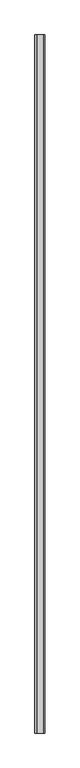
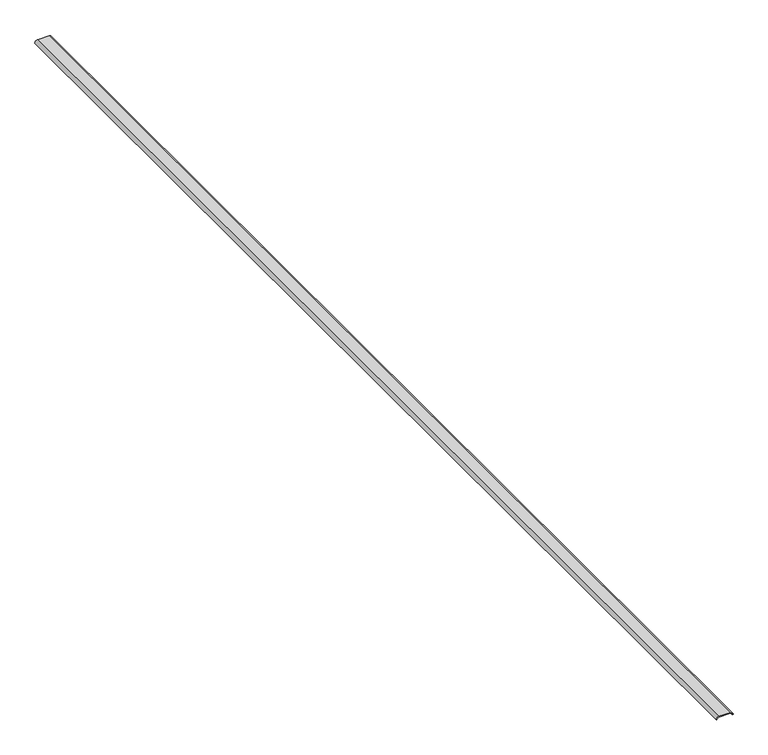
"""IFC4 building model written with IfcOpenShell, lengths in millimetres: proxy geometry, BEND PANEL004 6191 : BEND PANEL004 6191."""

import ifcopenshell
import ifcopenshell.guid

model = None  # the IFC model being written
_history = None  # IfcOwnerHistory: only IFC2X3 demands one
_inside = {}  # id of a spatial element -> (the spatial element, [elements in it])
_under = {}  # id of a project, library or spatial element -> (it, [spatial elements below it])
_declared = {}  # id of a project -> (the project, [libraries it declares])
_typed = {}  # id of a type object -> (the type object, [elements of that type])
_made_of = {}  # id of a material, layer set ... -> (it, [elements and type objects made of it])


def new_model(schema):
    """Start an empty IFC model of exactly this schema.

    Asked for "IFC4X3", IfcOpenShell would pick the latest addendum, in which some entities
    have other attributes; the version numbers below select the first issue.
    IFC2X3 requires an IfcOwnerHistory on every rooted entity: one is made here for all.
    """
    global model, _history
    if schema == "IFC4X3":
        model = ifcopenshell.file(schema_version=(4, 3, 0, 0))
    else:
        model = ifcopenshell.file(schema=schema)
    _inside.clear()
    _under.clear()
    _declared.clear()
    _typed.clear()
    _made_of.clear()
    _history = None
    if model.schema == "IFC2X3":
        org = make("IfcOrganization", Name="unknown")
        user = make(
            "IfcPersonAndOrganization",
            ThePerson=make("IfcPerson", FamilyName="unknown"),
            TheOrganization=org,
        )
        app = make(
            "IfcApplication",
            ApplicationDeveloper=org,
            Version="unknown",
            ApplicationFullName="unknown",
            ApplicationIdentifier="unknown",
        )
        _history = make(
            "IfcOwnerHistory",
            OwningUser=user,
            OwningApplication=app,
            ChangeAction="ADDED",
            CreationDate=0,
        )
    return model


def make(cls, **values):
    """One entity of the class cls with the attributes given. An attribute that is None is left unset."""
    return model.create_entity(
        cls, **{name: value for name, value in values.items() if value is not None}
    )


def rooted(cls, **values):
    """An entity with a GlobalId (a new one), such as an element, a storey or a relation."""
    return make(cls, GlobalId=ifcopenshell.guid.new(), OwnerHistory=_history, **values)


def si_unit(unit_type, name, prefix=None):
    """IfcSIUnit, for example si_unit("LENGTHUNIT", "METRE", prefix="MILLI")."""
    return make("IfcSIUnit", UnitType=unit_type, Prefix=prefix, Name=name)


def assignment(units):
    """IfcUnitAssignment: the units of a project."""
    return None if units is None else make("IfcUnitAssignment", Units=units)


def point(xyz):
    """IfcCartesianPoint."""
    return None if xyz is None else make("IfcCartesianPoint", Coordinates=xyz)


def direction(xyz):
    """IfcDirection."""
    return None if xyz is None else make("IfcDirection", DirectionRatios=xyz)


def frame(location, z_axis=None, x_axis=None):
    """IfcAxis2Placement3D, a coordinate frame: its origin and axes. An axis left out is left unset."""
    return make(
        "IfcAxis2Placement3D",
        Location=point(location),
        Axis=direction(z_axis),
        RefDirection=direction(x_axis),
    )


def frame_2d(location, x_axis=None):
    """IfcAxis2Placement2D, a coordinate frame in the plane: its origin and x axis."""
    return make(
        "IfcAxis2Placement2D", Location=point(location), RefDirection=direction(x_axis)
    )


def origin():
    """The frame at (0, 0, 0) with its axes left unset."""
    return frame((0.0, 0.0, 0.0))


def place(relative_to, where):
    """IfcLocalPlacement: puts the frame where relative to a parent placement (None: the world)."""
    return make(
        "IfcLocalPlacement", PlacementRelTo=relative_to, RelativePlacement=where
    )


def context(
    kind, dimensions, precision=None, world=None, true_north=None, identifier=None
):
    """IfcGeometricRepresentationContext, for example the 3D "Model" context."""
    return make(
        "IfcGeometricRepresentationContext",
        ContextIdentifier=identifier,
        ContextType=kind,
        CoordinateSpaceDimension=dimensions,
        Precision=precision,
        WorldCoordinateSystem=world,
        TrueNorth=true_north,
    )


def project(units=None, contexts=None):
    """IfcProject with its units and contexts."""
    return rooted(
        "IfcProject",
        Name="project",
        RepresentationContexts=contexts,
        UnitsInContext=assignment(units),
    )


def spatial(cls, under=None, at=None, **own):
    """A site, building, storey or space (cls), placed at a placement, below another one or the project."""
    s = rooted(cls, ObjectPlacement=at, **own)
    if under is not None:
        _under.setdefault(under.id(), (under, []))[1].append(s)
    return s


def polyline(points):
    """IfcPolyline through the points."""
    return make("IfcPolyline", Points=[point(p) for p in points])


def circle_curve(where, radius):
    """IfcCircle in the frame where."""
    return make("IfcCircle", Position=where, Radius=radius)


def trimmed(basis, trim1, trim2, sense, master):
    """IfcTrimmedCurve: the piece of a basis curve between two trims."""
    return make(
        "IfcTrimmedCurve",
        BasisCurve=basis,
        Trim1=trim1,
        Trim2=trim2,
        SenseAgreement=sense,
        MasterRepresentation=master,
    )


def segment(curve, same_sense, transition):
    """IfcCompositeCurveSegment."""
    return make(
        "IfcCompositeCurveSegment",
        Transition=transition,
        SameSense=same_sense,
        ParentCurve=curve,
    )


def composite_curve(segments, self_intersect=None):
    """IfcCompositeCurve: segments joined end to end."""
    return make("IfcCompositeCurve", Segments=segments, SelfIntersect=self_intersect)


def outline(outer, holes=None, kind="AREA"):
    """IfcArbitraryClosedProfileDef: a profile drawn as a closed curve; with holes, ...WithVoids."""
    if holes is None:
        return make("IfcArbitraryClosedProfileDef", ProfileType=kind, OuterCurve=outer)
    return make(
        "IfcArbitraryProfileDefWithVoids",
        ProfileType=kind,
        OuterCurve=outer,
        InnerCurves=holes,
    )


def extrude(swept, where, along, depth):
    """IfcExtrudedAreaSolid: the profile swept, set in the frame where, extruded along a direction by depth."""
    return make(
        "IfcExtrudedAreaSolid",
        SweptArea=swept,
        Position=where,
        ExtrudedDirection=direction(along),
        Depth=depth,
    )


def shape(context_of_items, identifier, shape_type, items):
    """IfcShapeRepresentation: the items that make up one representation, for example the "Body"."""
    return make(
        "IfcShapeRepresentation",
        ContextOfItems=context_of_items,
        RepresentationIdentifier=identifier,
        RepresentationType=shape_type,
        Items=items,
    )


def source(mapping_origin, context_of_items, identifier, shape_type, items):
    """IfcRepresentationMap: a shape defined once, which mapped items show again and again."""
    return make(
        "IfcRepresentationMap",
        MappingOrigin=mapping_origin,
        MappedRepresentation=shape(context_of_items, identifier, shape_type, items),
    )


def transform(
    local_origin,
    x_axis=None,
    y_axis=None,
    z_axis=None,
    scale=None,
    scale2=None,
    scale3=None,
    uniform=True,
):
    """IfcCartesianTransformationOperator3D, or its non-uniform kind. x_axis, y_axis, z_axis: its Axis1, 2, 3."""
    if uniform:
        return make(
            "IfcCartesianTransformationOperator3D",
            Axis1=direction(x_axis),
            Axis2=direction(y_axis),
            LocalOrigin=point(local_origin),
            Scale=scale,
            Axis3=direction(z_axis),
        )
    return make(
        "IfcCartesianTransformationOperator3DnonUniform",
        Axis1=direction(x_axis),
        Axis2=direction(y_axis),
        LocalOrigin=point(local_origin),
        Scale=scale,
        Axis3=direction(z_axis),
        Scale2=scale2,
        Scale3=scale3,
    )


def mapped(mapping_source, mapping_target):
    """IfcMappedItem: shows the shape of a source again, moved by a transform."""
    return make(
        "IfcMappedItem", MappingSource=mapping_source, MappingTarget=mapping_target
    )


def made_of(thing, what):
    """Note that an element or type object is made of a material, layer set ...; save() writes the relation."""
    if what is not None:
        _made_of.setdefault(what.id(), (what, []))[1].append(thing)
    return thing


def element(
    cls,
    number,
    at=None,
    inside=None,
    cuts=None,
    type_object=None,
    material=None,
    context=None,
    identifier="Body",
    shape_type=None,
    held_by="IfcProductDefinitionShape",
    body=None,
    shapes=None,
    **own,
):
    """One element of the class cls, such as IfcWall. Its Tag is "e" and its number.

    at: its placement. inside: the storey or other place that contains it. cuts: it is an
    opening in that element (IfcRelVoidsElement). A single representation is given by context,
    identifier, shape_type and body (its items); several are given by shapes. held_by: the class
    of the entity that holds the representations. save() writes the other relations.
    """
    e = rooted(cls, Tag="e%d" % number, ObjectPlacement=at, **own)
    if body is not None:
        shapes = [shape(context, identifier, shape_type, body)]
    if shapes is not None:
        e.Representation = make(held_by, Representations=shapes)
    if inside is not None:
        _inside.setdefault(inside.id(), (inside, []))[1].append(e)
    if cuts is not None:
        rooted(
            "IfcRelVoidsElement", RelatingBuildingElement=cuts, RelatedOpeningElement=e
        )
    if type_object is not None:
        _typed.setdefault(type_object.id(), (type_object, []))[1].append(e)
    return made_of(e, material)


def aggregate(whole, parts):
    """IfcRelAggregates: a whole, such as a stair, and the parts it consists of."""
    return rooted("IfcRelAggregates", RelatingObject=whole, RelatedObjects=parts)


def save(model, path):
    """Write the relations noted so far, then the file.

    IfcRelAggregates (storeys below a building ...), IfcRelContainedInSpatialStructure (elements
    in a storey), IfcRelDefinesByType, IfcRelAssociatesMaterial and IfcRelDeclares: one each for
    every whole, place, type object, material and project.
    """
    for whole, parts in _under.values():
        aggregate(whole, parts)
    for where, things in _inside.values():
        rooted(
            "IfcRelContainedInSpatialStructure",
            RelatedElements=things,
            RelatingStructure=where,
        )
    for kind, things in _typed.values():
        rooted("IfcRelDefinesByType", RelatedObjects=things, RelatingType=kind)
    for what, things in _made_of.values():
        rooted("IfcRelAssociatesMaterial", RelatedObjects=things, RelatingMaterial=what)
    for by, libraries in _declared.values():
        rooted("IfcRelDeclares", RelatingContext=by, RelatedDefinitions=libraries)
    model.write(path)


def generic_models_15d214a6(model_context):
    return source(origin(), model_context, "Body", "SweptSolid", [
        extrude(outline(composite_curve([segment(polyline([(42576.61192, 5858.4004637), (42576.61192, 5859.5910887)]), True, "CONTINUOUS"), segment(trimmed(circle_curve(frame_2d((42576.6119199, 5862.9993652)), 3.4082764), [point((42576.61192, 5859.5910887))], [point((42580.0201795, 5863.0100787))], True, "CARTESIAN"), True, "CONTINUOUS"), segment(polyline([(42580.0201795, 5863.0100787), (42580.0201963, 5882.3645691)]), True, "CONTINUOUS"), segment(trimmed(circle_curve(frame_2d((42576.6119199, 5882.3645721)), 3.4082764), [point((42580.0201963, 5882.3645691))], [point((42576.61192, 5885.7728485))], True, "CARTESIAN"), True, "CONTINUOUS"), segment(polyline([(42576.61192, 5885.7728485), (42576.61192, 5886.9634735)]), True, "CONTINUOUS"), segment(trimmed(circle_curve(frame_2d((42576.6119199, 5882.3645721)), 4.5989014), [point((42576.61192, 5886.9634735))], [point((42581.2108213, 5882.364568))], False, "CARTESIAN"), True, "CONTINUOUS"), segment(polyline([(42581.2108213, 5882.364568), (42581.2108045, 5863.0118181)]), True, "CONTINUOUS"), segment(trimmed(circle_curve(frame_2d((42576.6119199, 5862.9993652)), 4.5989014), [point((42581.2108045, 5863.0118181))], [point((42576.61192, 5858.4004637))], False, "CARTESIAN"), True, "CONTINUOUS")], self_intersect=False)), frame((0.0, -1052.8906574, 0.0), z_axis=(0.0, 1.0, 0.0), x_axis=(0.0, 0.0, 1.0)), (0.0, 0.0, 1.0), 1999.85),
    ])


if __name__ == "__main__":
    model = new_model("IFC4")
    model_context = context("Model", 3, world=origin())
    ifc_project = project(units=[si_unit("LENGTHUNIT", "METRE", prefix="MILLI")], contexts=[model_context])
    site = spatial("IfcSite", under=ifc_project)
    building = spatial("IfcBuilding", under=site)
    placement = place(None, origin())
    generic_models_shape = generic_models_15d214a6(model_context)
    element("IfcBuildingElementProxy", 1, Name="BEND PANEL004 6191 : BEND PANEL004 6191", ObjectType="BEND PANEL004 6191 : BEND PANEL004 6191", at=placement, inside=building, context=model_context, shape_type="MappedRepresentation", body=[
        mapped(generic_models_shape, transform((0.0, 0.0, 0.0), x_axis=(1.0, 0.0, 0.0), y_axis=(0.0, 1.0, 0.0), z_axis=(0.0, 0.0, 1.0))),
    ])
    save(model, "model.ifc")

# Revit data of these elements
# Type "BEND PANEL004 6191 : BEND PANEL004 6191"
#   NameOverride = "BEND PANEL004"
# Element 1 (IfcBuildingElementProxy, "BEND PANEL004 6191 : BEND PANEL004 6191")
#   Materials on its faces: "METAL PROFILE"
# Materials
#   "METAL PROFILE": class "Unassigned", colour RGB 128 128 128, transparency 0
